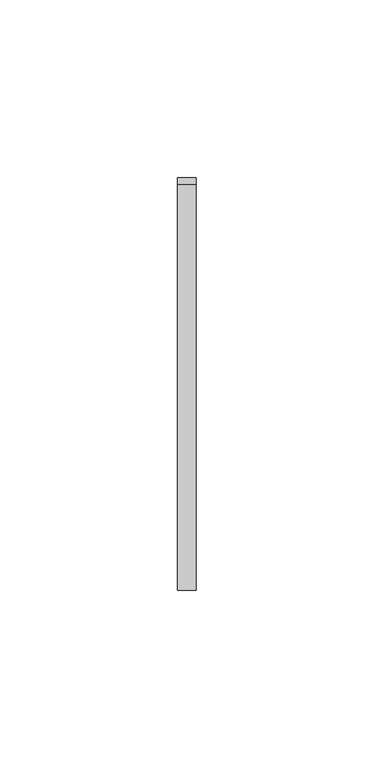
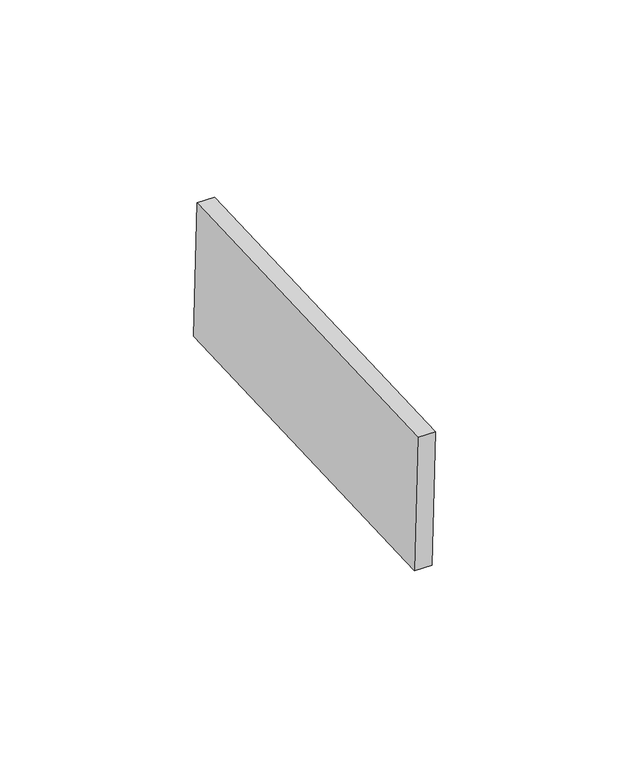
"""IFC4 building model written with IfcOpenShell, lengths in millimetres: proxy geometry, Inner panel:Inner panel:1:Inner panel:1 : Inner panel:Inner panel:300324:2:Inner panel:1:Inner panel:1 : Inner panel:Inner panel:300324:2 : Inner panel:Inner panel:1:Inner panel:1 : Inner panel:Inner panel:300324:300043:71 : Inner panel:Inner panel:1:Inner panel:1 : Inner panel:Inner panel:300324:2:Inner panel:1:Inner panel:1 : Inner panel:Inner panel:300324:2 : Inner panel:Inner panel:1:Inner panel:1 : Inner panel:Inner panel:300324:300043:308120."""

from ifc_helpers import new_model, si_unit, frame, origin, place, context, project, spatial, polyline, outline, extrude, source, transform, mapped, element, save


def generic_models_7cc6e8b7(model_context):
    return source(origin(), model_context, "Body", "SweptSolid", [
        extrude(outline(polyline([(0.0, -114.2999999), (0.0, 0.0), (5.2138089, 0.0), (5.2138089, -114.2999999), (0.0, -114.2999999)])), frame((593936.595117, -568168.273882, 8806.9397902), z_axis=(0.0, -0.04163054471215927, 0.9991330730923529), x_axis=(-1.0, 0.0, 0.0)), (0.0, 0.0, 1.0), 43.2233908),
    ])


if __name__ == "__main__":
    model = new_model("IFC4")
    model_context = context("Model", 3, world=origin())
    ifc_project = project(units=[si_unit("LENGTHUNIT", "METRE", prefix="MILLI")], contexts=[model_context])
    site = spatial("IfcSite", under=ifc_project)
    building = spatial("IfcBuilding", under=site)
    placement = place(None, origin())
    generic_models_shape = generic_models_7cc6e8b7(model_context)
    element("IfcBuildingElementProxy", 1, Name="Inner panel:Inner panel:1:Inner panel:1 : Inner panel:Inner panel:300324:2:Inner panel:1:Inner panel:1 : Inner panel:Inner panel:300324:2 : Inner panel:Inner panel:1:Inner panel:1 : Inner panel:Inner panel:300324:300043:71 : Inner panel:Inner panel:1:Inner panel:1 : Inner panel:Inner panel:300324:2:Inner panel:1:Inner panel:1 : Inner panel:Inner panel:300324:2 : Inner panel:Inner panel:1:Inner panel:1 : Inner panel:Inner panel:300324:300043:308120", ObjectType="Inner panel:Inner panel:1:Inner panel:1 : Inner panel:Inner panel:300324:2:Inner panel:1:Inner panel:1 : Inner panel:Inner panel:300324:2 : Inner panel:Inner panel:1:Inner panel:1 : Inner panel:Inner panel:300324:300043:71 : Inner panel:Inner panel:1:Inner panel:1 : Inner panel:Inner panel:300324:2:Inner panel:1:Inner panel:1 : Inner panel:Inner panel:300324:2 : Inner panel:Inner panel:1:Inner panel:1 : Inner panel:Inner panel:300324:300043:308120", at=placement, inside=building, context=model_context, shape_type="MappedRepresentation", body=[
        mapped(generic_models_shape, transform((0.0, 0.0, 0.0), x_axis=(1.0, 0.0, 0.0), y_axis=(0.0, 1.0, 0.0), z_axis=(0.0, 0.0, 1.0))),
    ])
    save(model, "model.ifc")

# Revit data of these elements
# Type "Inner panel:Inner panel:1:Inner panel:1 : Inner panel:Inner panel:300324:2:Inner panel:1:Inner panel:1 : Inner panel:Inner panel:300324:2 : Inner panel:Inner panel:1:Inner panel:1 : Inner panel:Inner panel:300324:300043:71 : Inner panel:Inner panel:1:Inner panel:1 : Inner panel:Inner panel:300324:2:Inner panel:1:Inner panel:1 : Inner panel:Inner panel:300324:2 : Inner panel:Inner panel:1:Inner panel:1 : Inner panel:Inner panel:300324:300043:308120"
#   NameOverride = "Inner panel:Inner panel:1:Inner panel:1 : Inner panel:Inner panel:300324:2:Inner panel:1:Inner panel:1 : Inner panel:Inner panel:300324:2 : Inner panel:Inner panel:1:Inner panel:1 : Inner panel:Inner panel:300324:300043:308120"
#   ObjectTypeOverride = "Inner panel:1:Inner panel:1 : Inner panel:Inner panel:300324:2 : Inner panel:Inner panel:1:Inner panel:1 : Inner panel:Inner panel:300324:300043"
#   Reference = "Inner panel"
#   Tag = "308120"
# Element 1 (IfcBuildingElementProxy, "Inner panel:Inner panel:1:Inner panel:1 : Inner panel:Inner panel:300324:2:Inner panel:1:Inner panel:1 : Inner panel:Inner panel:300324:2 : Inner panel:Inner panel:1:Inner panel:1 : Inner panel:Inner panel:300324:300043:71 : Inner panel:Inner panel:1:Inner panel:1 : Inner panel:Inner panel:300324:2:Inner panel:1:Inner panel:1 : Inner panel:Inner panel:300324:2 : Inner panel:Inner panel:1:Inner panel:1 : Inner panel:Inner panel:300324:300043:308120")
#   Materials on its faces: "SLIDING CLIP"
# Materials
#   "SLIDING CLIP": class "Generic", colour RGB 120 120 120, transparency 0, Cost = 0
